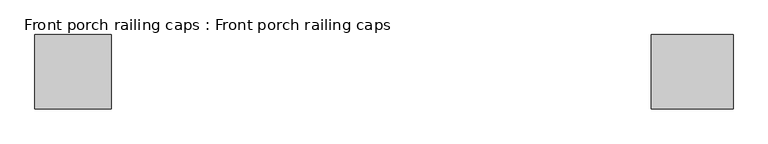
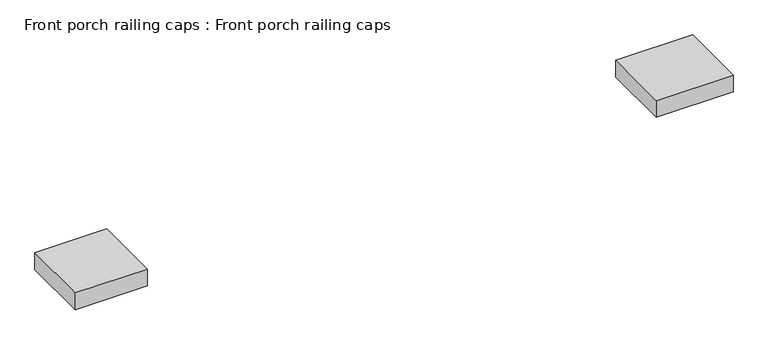
"""IFC4 building model written with IfcOpenShell, lengths in millimetres: furniture geometry, Front porch railing caps : Front porch railing caps."""

from ifc_helpers import new_model, si_unit, frame, origin, place, context, project, spatial, polyline, outline, extrude, source, transform, mapped, element, save


def front_porch_railing_caps_front_porch_railing_caps_115c7716(model_context):
    return source(origin(), model_context, "Body", "SweptSolid", [
        extrude(outline(polyline([(1143.8137312, 18746.8054342), (831.3027851, 18746.8054342), (831.3027851, 19051.6054342), (1143.8137312, 19051.6054342), (1143.8137312, 18746.8054342)])), frame((0.0, 0.0, 385.5962572), z_axis=(0.0, 0.0, 1.0), x_axis=(1.0, 0.0, 0.0)), (0.0, 0.0, 1.0), 77.3993939),
        extrude(outline(polyline([(3692.9770441, 19051.6054342), (3692.9770441, 18746.8054342), (3358.3899812, 18746.8054342), (3358.3899812, 19051.6054342), (3692.9770441, 19051.6054342)])), frame((0.0, 0.0, 385.5962572), z_axis=(0.0, 0.0, 1.0), x_axis=(1.0, 0.0, 0.0)), (0.0, 0.0, 1.0), 77.3993939),
    ])


if __name__ == "__main__":
    model = new_model("IFC4")
    model_context = context("Model", 3, world=origin())
    ifc_project = project(units=[si_unit("LENGTHUNIT", "METRE", prefix="MILLI")], contexts=[model_context])
    site = spatial("IfcSite", under=ifc_project)
    building = spatial("IfcBuilding", under=site)
    placement = place(None, origin())
    front_porch_railing_caps_front_porch_railing_caps_shape = front_porch_railing_caps_front_porch_railing_caps_115c7716(model_context)
    element("IfcFurniture", 1, ObjectType="Front porch railing caps : Front porch railing caps", at=placement, inside=building, context=model_context, shape_type="MappedRepresentation", body=[
        mapped(front_porch_railing_caps_front_porch_railing_caps_shape, transform((0.0, 0.0, 0.0), x_axis=(1.0, 0.0, 0.0), y_axis=(0.0, 1.0, 0.0), z_axis=(0.0, 0.0, 1.0))),
    ])
    save(model, "model.ifc")

# Revit data of these elements
# Type "Front porch railing caps : Front porch railing caps"
#   COBie.Type = no
# Element 1 (IfcFurniture, "Front porch railing caps : Front porch railing caps")
#   Materials on its faces: "Floor Stone"
# Materials
#   "Floor Stone": class "Stone", colour RGB 107 106 105, transparency 0, Cost = 0
